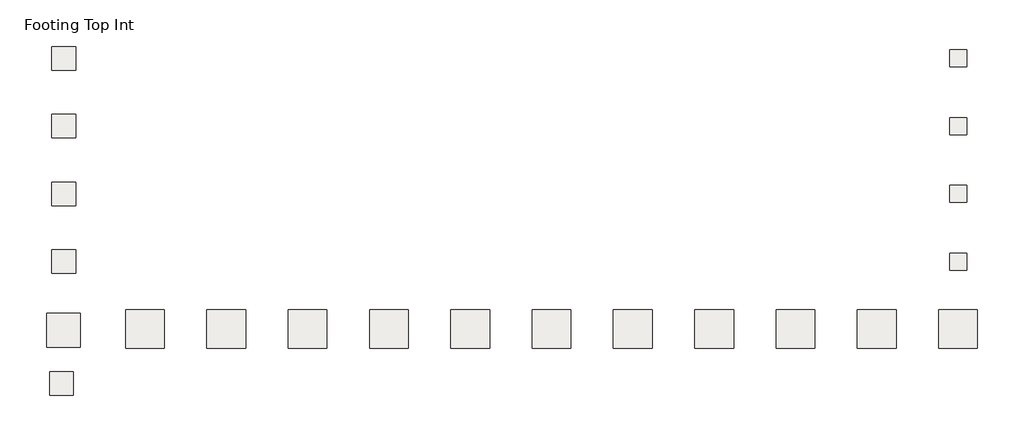
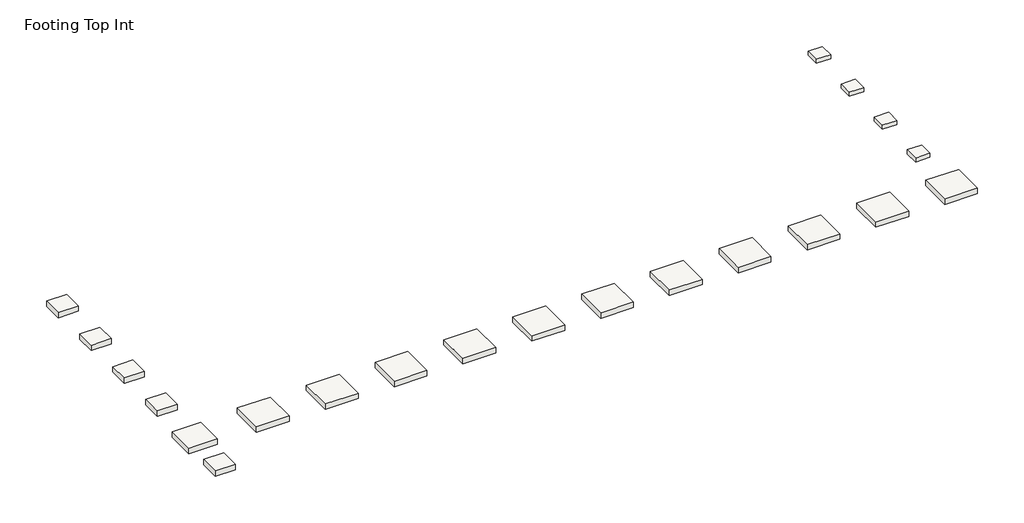
# One storey: 21 slabs.
"""IFC4 building model written with IfcOpenShell, lengths in millimetres."""

from ifc_helpers import new_model, si_unit, frame, origin, place, context, project, spatial, polyline, outline, extrude, faceted_brep, element, save

model = new_model("IFC4")

# Units and contexts
model_context = context("Model", 3, world=origin())
ifc_project = project(units=[si_unit("LENGTHUNIT", "METRE", prefix="MILLI")], contexts=[model_context])

# Site, building, storey
site = spatial("IfcSite", under=ifc_project)
building = spatial("IfcBuilding", under=site)
storey = spatial("IfcBuildingStorey", under=building, Name="Footing Top Int", Elevation=-304.8)

# Slabs
placement = place(None, origin())
element("IfcSlab", 1, ObjectType="Footing-Rectangular : F10", at=placement, inside=storey, context=model_context, shape_type="SweptSolid", body=[
    extrude(outline(polyline([(321699.0398264, -566249.8913841), (324747.0398264, -566249.8913841), (324747.0398264, -569297.8913841), (321699.0398264, -569297.8913841), (321699.0398264, -566249.8913841)])), frame((0.0, 0.0, -914.4), z_axis=(0.0, 0.0, 1.0), x_axis=(1.0, 0.0, 0.0)), (0.0, 0.0, 1.0), 609.6),
])
element("IfcSlab", 2, ObjectType="Footing-Rectangular : F11", at=placement, inside=storey, context=model_context, shape_type="SweptSolid", body=[
    extrude(outline(polyline([(328849.1398264, -565913.3414082), (332354.3398264, -565913.3414082), (332354.3398264, -569418.5414082), (328849.1398264, -569418.5414082), (328849.1398264, -565913.3414082)])), frame((0.0, 0.0, -914.4), z_axis=(0.0, 0.0, 1.0), x_axis=(1.0, 0.0, 0.0)), (0.0, 0.0, 1.0), 609.6),
])
element("IfcSlab", 3, ObjectType="Footing-Rectangular : F11", at=placement, inside=storey, context=model_context, shape_type="SweptSolid", body=[
    extrude(outline(polyline([(336202.4398264, -565913.3414082), (339707.6398264, -565913.3414082), (339707.6398264, -569418.5414082), (336202.4398264, -569418.5414082), (336202.4398264, -565913.3414082)])), frame((0.0, 0.0, -914.4), z_axis=(0.0, 0.0, 1.0), x_axis=(1.0, 0.0, 0.0)), (0.0, 0.0, 1.0), 609.6),
])
element("IfcSlab", 4, ObjectType="Footing-Rectangular : F11", at=placement, inside=storey, context=model_context, shape_type="SweptSolid", body=[
    extrude(outline(polyline([(343555.7398264, -565913.3414082), (347060.9398264, -565913.3414082), (347060.9398264, -569418.5414082), (343555.7398264, -569418.5414082), (343555.7398264, -565913.3414082)])), frame((0.0, 0.0, -914.4), z_axis=(0.0, 0.0, 1.0), x_axis=(1.0, 0.0, 0.0)), (0.0, 0.0, 1.0), 609.6),
])
element("IfcSlab", 5, ObjectType="Footing-Rectangular : F11", at=placement, inside=storey, context=model_context, shape_type="SweptSolid", body=[
    extrude(outline(polyline([(350909.0398264, -565913.3414082), (354414.2398264, -565913.3414082), (354414.2398264, -569418.5414082), (350909.0398264, -569418.5414082), (350909.0398264, -565913.3414082)])), frame((0.0, 0.0, -914.4), z_axis=(0.0, 0.0, 1.0), x_axis=(1.0, 0.0, 0.0)), (0.0, 0.0, 1.0), 609.6),
])
element("IfcSlab", 6, ObjectType="Footing-Rectangular : F11", at=placement, inside=storey, context=model_context, shape_type="SweptSolid", body=[
    extrude(outline(polyline([(358262.3398264, -565913.3414082), (361767.5398264, -565913.3414082), (361767.5398264, -569418.5414082), (358262.3398264, -569418.5414082), (358262.3398264, -565913.3414082)])), frame((0.0, 0.0, -914.4), z_axis=(0.0, 0.0, 1.0), x_axis=(1.0, 0.0, 0.0)), (0.0, 0.0, 1.0), 609.6),
])
element("IfcSlab", 7, ObjectType="Footing-Rectangular : F11", at=placement, inside=storey, context=model_context, shape_type="SweptSolid", body=[
    extrude(outline(polyline([(365615.6398264, -565913.3414082), (369120.8398264, -565913.3414082), (369120.8398264, -569418.5414082), (365615.6398264, -569418.5414082), (365615.6398264, -565913.3414082)])), frame((0.0, 0.0, -914.4), z_axis=(0.0, 0.0, 1.0), x_axis=(1.0, 0.0, 0.0)), (0.0, 0.0, 1.0), 609.6),
])
element("IfcSlab", 8, ObjectType="Footing-Rectangular : F11", at=placement, inside=storey, context=model_context, shape_type="SweptSolid", body=[
    extrude(outline(polyline([(372968.9398264, -565913.3414082), (376474.1398264, -565913.3414082), (376474.1398264, -569418.5414082), (372968.9398264, -569418.5414082), (372968.9398264, -565913.3414082)])), frame((0.0, 0.0, -914.4), z_axis=(0.0, 0.0, 1.0), x_axis=(1.0, 0.0, 0.0)), (0.0, 0.0, 1.0), 609.6),
])
element("IfcSlab", 9, ObjectType="Footing-Rectangular : F11", at=placement, inside=storey, context=model_context, shape_type="SweptSolid", body=[
    extrude(outline(polyline([(380322.2398264, -565913.3414082), (383827.4398264, -565913.3414082), (383827.4398264, -569418.5414082), (380322.2398264, -569418.5414082), (380322.2398264, -565913.3414082)])), frame((0.0, 0.0, -914.4), z_axis=(0.0, 0.0, 1.0), x_axis=(1.0, 0.0, 0.0)), (0.0, 0.0, 1.0), 609.6),
])
element("IfcSlab", 10, ObjectType="Footing-Rectangular : F11", at=placement, inside=storey, context=model_context, shape_type="SweptSolid", body=[
    extrude(outline(polyline([(387675.5398264, -565913.3414082), (391180.7398264, -565913.3414082), (391180.7398264, -569418.5414082), (387675.5398264, -569418.5414082), (387675.5398264, -565913.3414082)])), frame((0.0, 0.0, -914.4), z_axis=(0.0, 0.0, 1.0), x_axis=(1.0, 0.0, 0.0)), (0.0, 0.0, 1.0), 609.6),
])
element("IfcSlab", 11, ObjectType="Footing-Rectangular : F11", at=placement, inside=storey, context=model_context, shape_type="SweptSolid", body=[
    extrude(outline(polyline([(395028.8398264, -565913.3414082), (398534.0398264, -565913.3414082), (398534.0398264, -569418.5414082), (395028.8398264, -569418.5414082), (395028.8398264, -565913.3414082)])), frame((0.0, 0.0, -914.4), z_axis=(0.0, 0.0, 1.0), x_axis=(1.0, 0.0, 0.0)), (0.0, 0.0, 1.0), 609.6),
])
element("IfcSlab", 12, ObjectType="Footing-Rectangular : F11", at=placement, inside=storey, context=model_context, shape_type="SweptSolid", body=[
    extrude(outline(polyline([(402382.1398264, -565913.3414082), (405887.3398264, -565913.3414082), (405887.3398264, -569418.5414082), (402382.1398264, -569418.5414082), (402382.1398264, -565913.3414082)])), frame((0.0, 0.0, -914.4), z_axis=(0.0, 0.0, 1.0), x_axis=(1.0, 0.0, 0.0)), (0.0, 0.0, 1.0), 609.6),
])
element("IfcSlab", 13, ObjectType="Footing-Rectangular : F5", at=placement, inside=storey, context=model_context, shape_type="SweptSolid", body=[
    extrude(outline(polyline([(404896.7398264, -542418.3413841), (404896.7398264, -543942.3413841), (403372.7398264, -543942.3413841), (403372.7398264, -542418.3413841), (404896.7398264, -542418.3413841)])), frame((0.0, 0.0, -762.0), z_axis=(0.0, 0.0, 1.0), x_axis=(1.0, 0.0, 0.0)), (0.0, 0.0, 1.0), 457.2),
])
element("IfcSlab", 14, ObjectType="Footing-Rectangular : F5", at=placement, inside=storey, context=model_context, shape_type="SweptSolid", body=[
    extrude(outline(polyline([(404896.7398264, -548546.0913841), (404896.7398264, -550070.0913841), (403372.7398264, -550070.0913841), (403372.7398264, -548546.0913841), (404896.7398264, -548546.0913841)])), frame((0.0, 0.0, -762.0), z_axis=(0.0, 0.0, 1.0), x_axis=(1.0, 0.0, 0.0)), (0.0, 0.0, 1.0), 457.2),
])
element("IfcSlab", 15, ObjectType="Footing-Rectangular : F5", at=placement, inside=storey, context=model_context, shape_type="SweptSolid", body=[
    extrude(outline(polyline([(404896.7398264, -554673.8413841), (404896.7398264, -556197.8413841), (403372.7398264, -556197.8413841), (403372.7398264, -554673.8413841), (404896.7398264, -554673.8413841)])), frame((0.0, 0.0, -762.0), z_axis=(0.0, 0.0, 1.0), x_axis=(1.0, 0.0, 0.0)), (0.0, 0.0, 1.0), 457.2),
])
element("IfcSlab", 16, ObjectType="Footing-Rectangular : F5", at=placement, inside=storey, context=model_context, shape_type="SweptSolid", body=[
    extrude(outline(polyline([(404896.7398264, -560801.5913841), (404896.7398264, -562325.5913841), (403372.7398264, -562325.5913841), (403372.7398264, -560801.5913841), (404896.7398264, -560801.5913841)])), frame((0.0, 0.0, -762.0), z_axis=(0.0, 0.0, 1.0), x_axis=(1.0, 0.0, 0.0)), (0.0, 0.0, 1.0), 457.2),
])
element("IfcSlab", 17, ObjectType="Footing-Rectangular : F7", at=placement, inside=storey, context=model_context, shape_type="Brep", body=[
    faceted_brep([(324121.5648264, -571526.7413841, -304.8), (321987.9648264, -571526.7413841, -304.8), (321987.9648264, -572404.4391729, -304.8), (321987.9648264, -572810.8391729, -304.8), (321987.9648264, -573660.3413841, -304.8), (324121.5648264, -573660.3413841, -304.8), (324121.5648264, -571526.7413841, -914.4), (324121.5648264, -573660.3413841, -914.4), (321987.9648264, -573660.3413841, -914.4), (321987.9648264, -571526.7413841, -914.4)], [[[0, 1, 2, 3, 4, 5]], [[6, 7, 8, 9]], [[1, 0, 6, 9]], [[4, 3, 2, 1, 9, 8]], [[5, 4, 8, 7]], [[0, 5, 7, 6]]]),
])
element("IfcSlab", 18, ObjectType="Footing-Rectangular : F7", at=placement, inside=storey, context=model_context, shape_type="SweptSolid", body=[
    extrude(outline(polyline([(324324.7648264, -542113.5413841), (324324.7648264, -544247.1413841), (322191.1648264, -544247.1413841), (322191.1648264, -542113.5413841), (324324.7648264, -542113.5413841)])), frame((0.0, 0.0, -914.4), z_axis=(0.0, 0.0, 1.0), x_axis=(1.0, 0.0, 0.0)), (0.0, 0.0, 1.0), 609.6),
])
element("IfcSlab", 19, ObjectType="Footing-Rectangular : F7", at=placement, inside=storey, context=model_context, shape_type="SweptSolid", body=[
    extrude(outline(polyline([(324324.7648264, -548241.2913841), (324324.7648264, -550374.8913841), (322191.1648264, -550374.8913841), (322191.1648264, -548241.2913841), (324324.7648264, -548241.2913841)])), frame((0.0, 0.0, -914.4), z_axis=(0.0, 0.0, 1.0), x_axis=(1.0, 0.0, 0.0)), (0.0, 0.0, 1.0), 609.6),
])
element("IfcSlab", 20, ObjectType="Footing-Rectangular : F7", at=placement, inside=storey, context=model_context, shape_type="SweptSolid", body=[
    extrude(outline(polyline([(324324.7648264, -554369.0413841), (324324.7648264, -556502.6413841), (322191.1648264, -556502.6413841), (322191.1648264, -554369.0413841), (324324.7648264, -554369.0413841)])), frame((0.0, 0.0, -914.4), z_axis=(0.0, 0.0, 1.0), x_axis=(1.0, 0.0, 0.0)), (0.0, 0.0, 1.0), 609.6),
])
element("IfcSlab", 21, ObjectType="Footing-Rectangular : F7", at=placement, inside=storey, context=model_context, shape_type="SweptSolid", body=[
    extrude(outline(polyline([(324324.7648264, -560496.7913841), (324324.7648264, -562630.3913841), (322191.1648264, -562630.3913841), (322191.1648264, -560496.7913841), (324324.7648264, -560496.7913841)])), frame((0.0, 0.0, -914.4), z_axis=(0.0, 0.0, 1.0), x_axis=(1.0, 0.0, 0.0)), (0.0, 0.0, 1.0), 609.6),
])

save(model, "model.ifc")

# Revit data of these elements
# Type "Footing-Rectangular : F10"
#   Assembly Code = "A1010100"
#   Width = 10' - 0"
#   Length = 10' - 0"
#   Thickness = 2' - 0"
#   Structural Material [instance default] = CONCRETE FOOTING - SEE STRUCT DWGS.
# Type "Footing-Rectangular : F11"
#   Assembly Code = "A1010100"
#   Width = 11' - 6"
#   Length = 11' - 6"
#   Thickness = 2' - 0"
#   Structural Material [instance default] = CONCRETE FOOTING - SEE STRUCT DWGS.
# Type "Footing-Rectangular : F5"
#   Assembly Code = "A1010100"
#   Width = 5' - 0"
#   Length = 5' - 0"
#   Thickness = 1' - 6"
#   Structural Material [instance default] = CONCRETE FOOTING - SEE STRUCT DWGS.
# Type "Footing-Rectangular : F7"
#   Assembly Code = "A1010100"
#   Width = 7' - 0"
#   Length = 7' - 0"
#   Thickness = 2' - 0"
#   Structural Material [instance default] = CONCRETE FOOTING - SEE STRUCT DWGS.
# Element 1 (IfcSlab, "Footing-Rectangular : F10")
#   Comments = ""
#   Structural Material = CONCRETE FOOTING - SEE STRUCT DWGS.
#   Phase Created = New Construction
#   Materials on its faces: "CONCRETE FOOTING - SEE STRUCT DWGS."
# Elements 2, 3, 4, 5, 6, 7, 8, 9, 10, 11, 12 (IfcSlab, "Footing-Rectangular : F11")
#   Comments = ""
#   Structural Material = CONCRETE FOOTING - SEE STRUCT DWGS.
#   Phase Created = New Construction
#   Materials on its faces: "CONCRETE FOOTING - SEE STRUCT DWGS."
# Elements 13, 14, 15, 16 (IfcSlab, "Footing-Rectangular : F5")
#   Comments = ""
#   Structural Material = CONCRETE FOOTING - SEE STRUCT DWGS.
#   Phase Created = New Construction
#   Materials on its faces: "CONCRETE FOOTING - SEE STRUCT DWGS."
# Elements 17, 18, 19, 20, 21 (IfcSlab, "Footing-Rectangular : F7")
#   Comments = ""
#   Structural Material = CONCRETE FOOTING - SEE STRUCT DWGS.
#   Phase Created = New Construction
#   Materials on its faces: "CONCRETE FOOTING - SEE STRUCT DWGS."
# Materials
#   "CONCRETE FOOTING - SEE STRUCT DWGS.": class "Concrete", colour RGB 192 192 192, transparency 0, Description = "Cast-in-place concrete", Cost = 0
